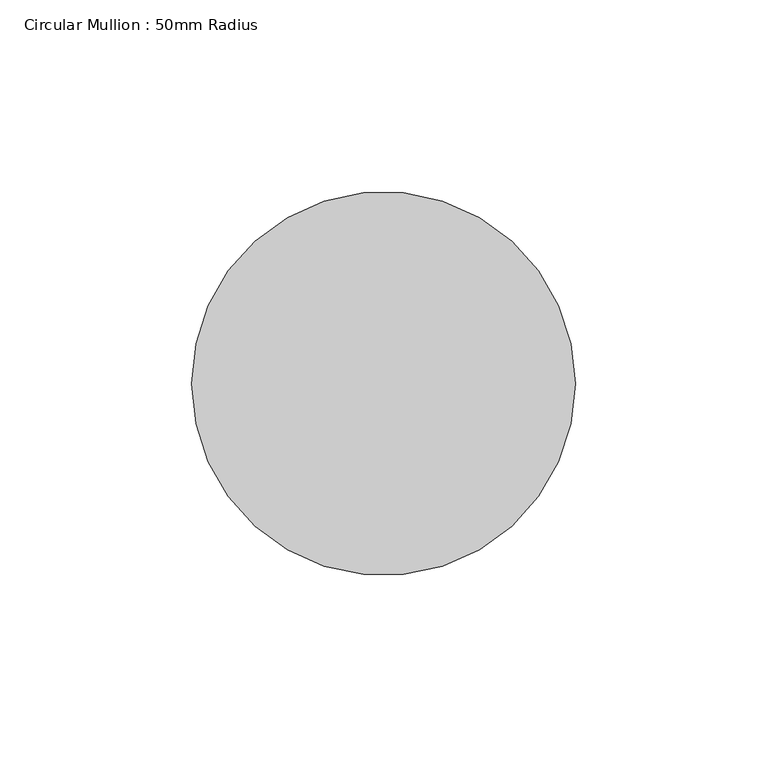
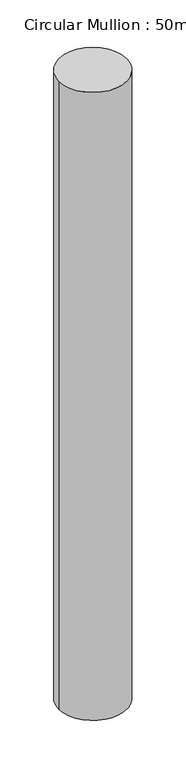
"""IFC4 building model written with IfcOpenShell, lengths in millimetres: member geometry, Circular Mullion : 50mm Radius."""

from ifc_helpers import new_model, si_unit, point, frame, origin, origin_2d, place, context, project, spatial, circle_curve, trimmed, segment, composite_curve, outline, extrude, source, transform, mapped, element, save


def circular_mullion_50mm_radius_51189e92(model_context):
    return source(origin(), model_context, "Body", "SweptSolid", [
        extrude(outline(composite_curve([segment(trimmed(circle_curve(origin_2d(), 50.0), [point((50.0, 0.0))], [point((-50.0, 0.0))], False, "CARTESIAN"), True, "CONTINUOUS"), segment(trimmed(circle_curve(origin_2d(), 50.0), [point((-50.0, 0.0))], [point((50.0, 0.0))], False, "CARTESIAN"), True, "CONTINUOUS")], self_intersect=False)), frame((0.0, 0.0, -977.0422355), z_axis=(0.0, 0.0, 1.0), x_axis=(1.0, 0.0, 0.0)), (0.0, 0.0, 1.0), 977.0422355),
    ])


if __name__ == "__main__":
    model = new_model("IFC4")
    model_context = context("Model", 3, world=origin())
    ifc_project = project(units=[si_unit("LENGTHUNIT", "METRE", prefix="MILLI")], contexts=[model_context])
    site = spatial("IfcSite", under=ifc_project)
    building = spatial("IfcBuilding", under=site)
    placement = place(None, origin())
    circular_mullion_50mm_radius_shape = circular_mullion_50mm_radius_51189e92(model_context)
    element("IfcMember", 1, ObjectType="Circular Mullion : 50mm Radius", at=placement, inside=building, context=model_context, shape_type="MappedRepresentation", body=[
        mapped(circular_mullion_50mm_radius_shape, transform((0.0, 0.0, 0.0), x_axis=(1.0, 0.0, 0.0), y_axis=(0.0, 1.0, 0.0), z_axis=(0.0, 0.0, 1.0))),
    ])
    save(model, "model.ifc")

# Revit data of these elements
# Type "Circular Mullion : 50mm Radius"
#   built-in parameter 1007350 = 0.164042 (stored number, unit not read)
# Element 1 (IfcMember, "Circular Mullion : 50mm Radius")
#   Materials on its faces: "Aluminium"
# Materials
#   "Aluminium": class "Metal", colour RGB 247 247 247, transparency 0, Description = "Aluminium 6061", Cost = 0
